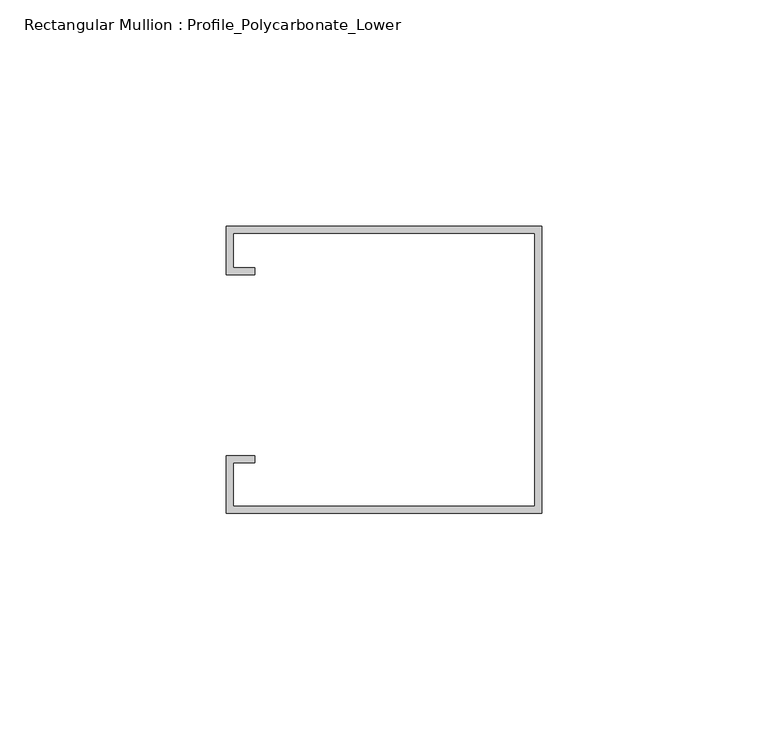
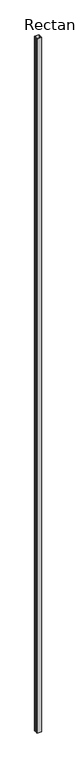
"""IFC4 building model written with IfcOpenShell, lengths in millimetres: member geometry, Rectangular Mullion : Profile_Polycarbonate_Lower."""

import ifcopenshell
import ifcopenshell.guid

model = None  # the IFC model being written
_history = None  # IfcOwnerHistory: only IFC2X3 demands one
_inside = {}  # id of a spatial element -> (the spatial element, [elements in it])
_under = {}  # id of a project, library or spatial element -> (it, [spatial elements below it])
_declared = {}  # id of a project -> (the project, [libraries it declares])
_typed = {}  # id of a type object -> (the type object, [elements of that type])
_made_of = {}  # id of a material, layer set ... -> (it, [elements and type objects made of it])


def new_model(schema):
    """Start an empty IFC model of exactly this schema.

    Asked for "IFC4X3", IfcOpenShell would pick the latest addendum, in which some entities
    have other attributes; the version numbers below select the first issue.
    IFC2X3 requires an IfcOwnerHistory on every rooted entity: one is made here for all.
    """
    global model, _history
    if schema == "IFC4X3":
        model = ifcopenshell.file(schema_version=(4, 3, 0, 0))
    else:
        model = ifcopenshell.file(schema=schema)
    _inside.clear()
    _under.clear()
    _declared.clear()
    _typed.clear()
    _made_of.clear()
    _history = None
    if model.schema == "IFC2X3":
        org = make("IfcOrganization", Name="unknown")
        user = make(
            "IfcPersonAndOrganization",
            ThePerson=make("IfcPerson", FamilyName="unknown"),
            TheOrganization=org,
        )
        app = make(
            "IfcApplication",
            ApplicationDeveloper=org,
            Version="unknown",
            ApplicationFullName="unknown",
            ApplicationIdentifier="unknown",
        )
        _history = make(
            "IfcOwnerHistory",
            OwningUser=user,
            OwningApplication=app,
            ChangeAction="ADDED",
            CreationDate=0,
        )
    return model


def make(cls, **values):
    """One entity of the class cls with the attributes given. An attribute that is None is left unset."""
    return model.create_entity(
        cls, **{name: value for name, value in values.items() if value is not None}
    )


def rooted(cls, **values):
    """An entity with a GlobalId (a new one), such as an element, a storey or a relation."""
    return make(cls, GlobalId=ifcopenshell.guid.new(), OwnerHistory=_history, **values)


def si_unit(unit_type, name, prefix=None):
    """IfcSIUnit, for example si_unit("LENGTHUNIT", "METRE", prefix="MILLI")."""
    return make("IfcSIUnit", UnitType=unit_type, Prefix=prefix, Name=name)


def assignment(units):
    """IfcUnitAssignment: the units of a project."""
    return None if units is None else make("IfcUnitAssignment", Units=units)


def point(xyz):
    """IfcCartesianPoint."""
    return None if xyz is None else make("IfcCartesianPoint", Coordinates=xyz)


def direction(xyz):
    """IfcDirection."""
    return None if xyz is None else make("IfcDirection", DirectionRatios=xyz)


def frame(location, z_axis=None, x_axis=None):
    """IfcAxis2Placement3D, a coordinate frame: its origin and axes. An axis left out is left unset."""
    return make(
        "IfcAxis2Placement3D",
        Location=point(location),
        Axis=direction(z_axis),
        RefDirection=direction(x_axis),
    )


def origin():
    """The frame at (0, 0, 0) with its axes left unset."""
    return frame((0.0, 0.0, 0.0))


def place(relative_to, where):
    """IfcLocalPlacement: puts the frame where relative to a parent placement (None: the world)."""
    return make(
        "IfcLocalPlacement", PlacementRelTo=relative_to, RelativePlacement=where
    )


def context(
    kind, dimensions, precision=None, world=None, true_north=None, identifier=None
):
    """IfcGeometricRepresentationContext, for example the 3D "Model" context."""
    return make(
        "IfcGeometricRepresentationContext",
        ContextIdentifier=identifier,
        ContextType=kind,
        CoordinateSpaceDimension=dimensions,
        Precision=precision,
        WorldCoordinateSystem=world,
        TrueNorth=true_north,
    )


def project(units=None, contexts=None):
    """IfcProject with its units and contexts."""
    return rooted(
        "IfcProject",
        Name="project",
        RepresentationContexts=contexts,
        UnitsInContext=assignment(units),
    )


def spatial(cls, under=None, at=None, **own):
    """A site, building, storey or space (cls), placed at a placement, below another one or the project."""
    s = rooted(cls, ObjectPlacement=at, **own)
    if under is not None:
        _under.setdefault(under.id(), (under, []))[1].append(s)
    return s


def polyline(points):
    """IfcPolyline through the points."""
    return make("IfcPolyline", Points=[point(p) for p in points])


def outline(outer, holes=None, kind="AREA"):
    """IfcArbitraryClosedProfileDef: a profile drawn as a closed curve; with holes, ...WithVoids."""
    if holes is None:
        return make("IfcArbitraryClosedProfileDef", ProfileType=kind, OuterCurve=outer)
    return make(
        "IfcArbitraryProfileDefWithVoids",
        ProfileType=kind,
        OuterCurve=outer,
        InnerCurves=holes,
    )


def extrude(swept, where, along, depth):
    """IfcExtrudedAreaSolid: the profile swept, set in the frame where, extruded along a direction by depth."""
    return make(
        "IfcExtrudedAreaSolid",
        SweptArea=swept,
        Position=where,
        ExtrudedDirection=direction(along),
        Depth=depth,
    )


def shape(context_of_items, identifier, shape_type, items):
    """IfcShapeRepresentation: the items that make up one representation, for example the "Body"."""
    return make(
        "IfcShapeRepresentation",
        ContextOfItems=context_of_items,
        RepresentationIdentifier=identifier,
        RepresentationType=shape_type,
        Items=items,
    )


def source(mapping_origin, context_of_items, identifier, shape_type, items):
    """IfcRepresentationMap: a shape defined once, which mapped items show again and again."""
    return make(
        "IfcRepresentationMap",
        MappingOrigin=mapping_origin,
        MappedRepresentation=shape(context_of_items, identifier, shape_type, items),
    )


def transform(
    local_origin,
    x_axis=None,
    y_axis=None,
    z_axis=None,
    scale=None,
    scale2=None,
    scale3=None,
    uniform=True,
):
    """IfcCartesianTransformationOperator3D, or its non-uniform kind. x_axis, y_axis, z_axis: its Axis1, 2, 3."""
    if uniform:
        return make(
            "IfcCartesianTransformationOperator3D",
            Axis1=direction(x_axis),
            Axis2=direction(y_axis),
            LocalOrigin=point(local_origin),
            Scale=scale,
            Axis3=direction(z_axis),
        )
    return make(
        "IfcCartesianTransformationOperator3DnonUniform",
        Axis1=direction(x_axis),
        Axis2=direction(y_axis),
        LocalOrigin=point(local_origin),
        Scale=scale,
        Axis3=direction(z_axis),
        Scale2=scale2,
        Scale3=scale3,
    )


def mapped(mapping_source, mapping_target):
    """IfcMappedItem: shows the shape of a source again, moved by a transform."""
    return make(
        "IfcMappedItem", MappingSource=mapping_source, MappingTarget=mapping_target
    )


def made_of(thing, what):
    """Note that an element or type object is made of a material, layer set ...; save() writes the relation."""
    if what is not None:
        _made_of.setdefault(what.id(), (what, []))[1].append(thing)
    return thing


def element(
    cls,
    number,
    at=None,
    inside=None,
    cuts=None,
    type_object=None,
    material=None,
    context=None,
    identifier="Body",
    shape_type=None,
    held_by="IfcProductDefinitionShape",
    body=None,
    shapes=None,
    **own,
):
    """One element of the class cls, such as IfcWall. Its Tag is "e" and its number.

    at: its placement. inside: the storey or other place that contains it. cuts: it is an
    opening in that element (IfcRelVoidsElement). A single representation is given by context,
    identifier, shape_type and body (its items); several are given by shapes. held_by: the class
    of the entity that holds the representations. save() writes the other relations.
    """
    e = rooted(cls, Tag="e%d" % number, ObjectPlacement=at, **own)
    if body is not None:
        shapes = [shape(context, identifier, shape_type, body)]
    if shapes is not None:
        e.Representation = make(held_by, Representations=shapes)
    if inside is not None:
        _inside.setdefault(inside.id(), (inside, []))[1].append(e)
    if cuts is not None:
        rooted(
            "IfcRelVoidsElement", RelatingBuildingElement=cuts, RelatedOpeningElement=e
        )
    if type_object is not None:
        _typed.setdefault(type_object.id(), (type_object, []))[1].append(e)
    return made_of(e, material)


def aggregate(whole, parts):
    """IfcRelAggregates: a whole, such as a stair, and the parts it consists of."""
    return rooted("IfcRelAggregates", RelatingObject=whole, RelatedObjects=parts)


def save(model, path):
    """Write the relations noted so far, then the file.

    IfcRelAggregates (storeys below a building ...), IfcRelContainedInSpatialStructure (elements
    in a storey), IfcRelDefinesByType, IfcRelAssociatesMaterial and IfcRelDeclares: one each for
    every whole, place, type object, material and project.
    """
    for whole, parts in _under.values():
        aggregate(whole, parts)
    for where, things in _inside.values():
        rooted(
            "IfcRelContainedInSpatialStructure",
            RelatedElements=things,
            RelatingStructure=where,
        )
    for kind, things in _typed.values():
        rooted("IfcRelDefinesByType", RelatedObjects=things, RelatingType=kind)
    for what, things in _made_of.values():
        rooted("IfcRelAssociatesMaterial", RelatedObjects=things, RelatingMaterial=what)
    for by, libraries in _declared.values():
        rooted("IfcRelDeclares", RelatingContext=by, RelatedDefinitions=libraries)
    model.write(path)


def rectangular_mullion_profile_polycarbonate_lower_fbcf21d4(model_context):
    return source(origin(), model_context, "Body", "SweptSolid", [
        extrude(outline(polyline([(0.0, -32.7), (-69.85, -32.7), (-69.85, -20.0), (-63.5, -20.0), (-63.5, -21.5875), (-68.2625, -21.5875), (-68.2625, -31.1125), (-1.5875, -31.1125), (-1.5875, 29.2125), (-68.2625, 29.2125), (-68.2625, 21.5875), (-63.5, 21.5875), (-63.5, 20.0), (-69.85, 20.0), (-69.85, 30.8), (0.0, 30.8), (0.0, -32.7)])), frame((0.0, 0.0, -11717.3375), z_axis=(0.0, 0.0, 1.0), x_axis=(1.0, 0.0, 0.0)), (0.0, 0.0, 1.0), 11717.3375),
    ])


if __name__ == "__main__":
    model = new_model("IFC4")
    model_context = context("Model", 3, world=origin())
    ifc_project = project(units=[si_unit("LENGTHUNIT", "METRE", prefix="MILLI")], contexts=[model_context])
    site = spatial("IfcSite", under=ifc_project)
    building = spatial("IfcBuilding", under=site)
    placement = place(None, origin())
    rectangular_mullion_profile_polycarbonate_lower_shape = rectangular_mullion_profile_polycarbonate_lower_fbcf21d4(model_context)
    element("IfcMember", 1, ObjectType="Rectangular Mullion : Profile_Polycarbonate_Lower", at=placement, inside=building, context=model_context, shape_type="MappedRepresentation", body=[
        mapped(rectangular_mullion_profile_polycarbonate_lower_shape, transform((0.0, 0.0, 0.0), x_axis=(1.0, 0.0, 0.0), y_axis=(0.0, 1.0, 0.0), z_axis=(0.0, 0.0, 1.0))),
    ])
    save(model, "model.ifc")

# Revit data of these elements
# Type "Rectangular Mullion : Profile_Polycarbonate_Lower"
#   built-in parameter 1007322 = 0.208333 (stored number, unit not read)
#   built-in parameter 1007321 = 0 (stored number, unit not read)
#   built-in parameter 1007320 = 0.00520833 (stored number, unit not read)
